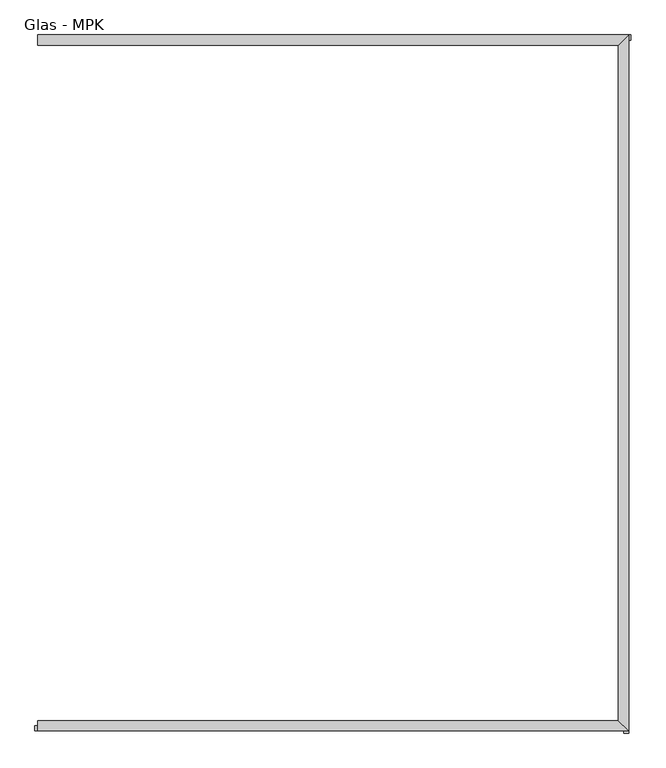
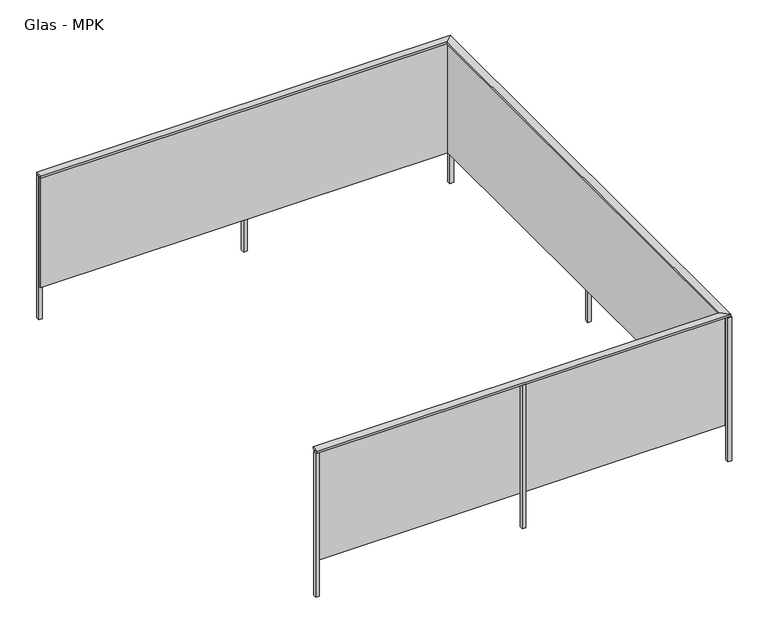
"""IFC4 building model written with IfcOpenShell, lengths in millimetres: railing geometry, Glas - MPK."""

from ifc_helpers import new_model, si_unit, frame, origin, place, context, project, spatial, polyline, outline, extrude, faceted_brep, source, transform, mapped, element, save


def glas_mpk_c28c6285(model_context):
    return source(origin(), model_context, "Body", "SolidModel", [
        faceted_brep([(29194.1667192, -1196.642277, 3843.2628643), (29194.1667192, -1246.642277, 3843.2628643), (29194.1667192, -1246.642277, 3856.7371357), (29194.1667192, -1196.642277, 3856.7371357), (32034.1667192, -1196.642277, 3843.2628643), (31984.1667192, -1246.642277, 3843.2628643), (31984.1667192, -1246.642277, 3856.7371357), (32034.1667192, -1196.642277, 3856.7371357), (32034.1667192, -4537.3716232, 3843.2628643), (31984.1667192, -4487.3716232, 3843.2628643), (31984.1667192, -4487.3716232, 3856.7371357), (32034.1667192, -4537.3716232, 3856.7371357), (29194.1667192, -4537.3716232, 3843.2628643), (29194.1667192, -4537.3716232, 3856.7371357), (29194.1667192, -4487.3716232, 3856.7371357), (29194.1667192, -4487.3716232, 3843.2628643)], [[[0, 1, 2, 3]], [[1, 0, 4, 5]], [[2, 1, 5, 6]], [[3, 2, 6, 7]], [[0, 3, 7, 4]], [[5, 4, 8, 9]], [[6, 5, 9, 10]], [[7, 6, 10, 11]], [[4, 7, 11, 8]], [[12, 13, 14, 15]], [[9, 8, 12, 15]], [[10, 9, 15, 14]], [[11, 10, 14, 13]], [[8, 11, 13, 12]]]),
        faceted_brep([(29194.1667192, -1236.642277, 3842.8769824), (29194.1667192, -1222.4501531, 3842.8769824), (29194.1667192, -1222.4501531, 3042.8769824), (29194.1667192, -1236.642277, 3042.8769824), (31994.1667192, -1236.642277, 3842.8769824), (32008.3588432, -1222.4501531, 3842.8769824), (32008.3588432, -1222.4501531, 3042.8769824), (31994.1667192, -1236.642277, 3042.8769824), (31994.1667192, -4497.3716232, 3842.8769824), (32008.3588432, -4511.5637472, 3842.8769824), (32008.3588432, -4511.5637472, 3042.8769824), (31994.1667192, -4497.3716232, 3042.8769824), (29194.1667192, -4497.3716232, 3842.8769824), (29194.1667192, -4497.3716232, 3042.8769824), (29194.1667192, -4511.5637472, 3042.8769824), (29194.1667192, -4511.5637472, 3842.8769824)], [[[0, 1, 2, 3]], [[1, 0, 4, 5]], [[2, 1, 5, 6]], [[3, 2, 6, 7]], [[0, 3, 7, 4]], [[5, 4, 8, 9]], [[6, 5, 9, 10]], [[7, 6, 10, 11]], [[4, 7, 11, 8]], [[12, 13, 14, 15]], [[9, 8, 12, 15]], [[10, 9, 15, 14]], [[11, 10, 14, 13]], [[8, 11, 13, 12]]]),
        extrude(outline(polyline([(30625.4167192, -4512.3716232), (30625.4167192, -4537.3716232), (30600.4167192, -4537.3716232), (30600.4167192, -4512.3716232), (30625.4167192, -4512.3716232)])), frame((0.0, 0.0, 2800.0), z_axis=(0.0, 0.0, 1.0), x_axis=(1.0, 0.0, 0.0)), (0.0, 0.0, 1.0), 1043.2628643),
        extrude(outline(polyline([(32009.1667192, -2854.5069501), (32034.1667192, -2854.5069501), (32034.1667192, -2879.5069501), (32009.1667192, -2879.5069501), (32009.1667192, -2854.5069501)])), frame((0.0, 0.0, 2800.0), z_axis=(0.0, 0.0, 1.0), x_axis=(1.0, 0.0, 0.0)), (0.0, 0.0, 1.0), 1043.2628643),
        extrude(outline(polyline([(30600.4167192, -1221.642277), (30600.4167192, -1196.642277), (30625.4167192, -1196.642277), (30625.4167192, -1221.642277), (30600.4167192, -1221.642277)])), frame((0.0, 0.0, 2800.0), z_axis=(0.0, 0.0, 1.0), x_axis=(1.0, 0.0, 0.0)), (0.0, 0.0, 1.0), 1043.2628643),
        extrude(outline(polyline([(32009.1667192, -4522.3716232), (32034.1667192, -4522.3716232), (32034.1667192, -4547.3716232), (32009.1667192, -4547.3716232), (32009.1667192, -4522.3716232)])), frame((0.0, 0.0, 2800.0), z_axis=(0.0, 0.0, 1.0), x_axis=(1.0, 0.0, 0.0)), (0.0, 0.0, 1.0), 1043.2628643),
        extrude(outline(polyline([(32019.1667192, -1221.642277), (32019.1667192, -1196.642277), (32044.1667192, -1196.642277), (32044.1667192, -1221.642277), (32019.1667192, -1221.642277)])), frame((0.0, 0.0, 2800.0), z_axis=(0.0, 0.0, 1.0), x_axis=(1.0, 0.0, 0.0)), (0.0, 0.0, 1.0), 1043.2628643),
        extrude(outline(polyline([(29206.6667192, -4512.3716232), (29206.6667192, -4537.3716232), (29181.6667192, -4537.3716232), (29181.6667192, -4512.3716232), (29206.6667192, -4512.3716232)])), frame((0.0, 0.0, 2800.0), z_axis=(0.0, 0.0, 1.0), x_axis=(1.0, 0.0, 0.0)), (0.0, 0.0, 1.0), 1043.2628643),
        extrude(outline(polyline([(29194.1667192, -1221.642277), (29194.1667192, -1196.642277), (29219.1667192, -1196.642277), (29219.1667192, -1221.642277), (29194.1667192, -1221.642277)])), frame((0.0, 0.0, 2800.0), z_axis=(0.0, 0.0, 1.0), x_axis=(1.0, 0.0, 0.0)), (0.0, 0.0, 1.0), 1043.2628643),
    ])


if __name__ == "__main__":
    model = new_model("IFC4")
    model_context = context("Model", 3, world=origin())
    ifc_project = project(units=[si_unit("LENGTHUNIT", "METRE", prefix="MILLI")], contexts=[model_context])
    site = spatial("IfcSite", under=ifc_project)
    building = spatial("IfcBuilding", under=site)
    placement = place(None, origin())
    glas_mpk_shape = glas_mpk_c28c6285(model_context)
    element("IfcRailing", 1, ObjectType="Glas - MPK", at=placement, inside=building, context=model_context, shape_type="MappedRepresentation", body=[
        mapped(glas_mpk_shape, transform((0.0, 0.0, 0.0), x_axis=(1.0, 0.0, 0.0), y_axis=(0.0, 1.0, 0.0), z_axis=(0.0, 0.0, 1.0))),
    ])
    save(model, "model.ifc")

# Revit data of these elements
# Element 1 (IfcRailing, "Glas - MPK")
#   Materials on its faces: "Metal - Aluminum", "Window - Glass"
# Materials
#   "Metal - Aluminum": class "Unassigned", colour RGB 247 247 247, transparency 0, Comments = "Rendering appearance not upgraded "
#   "Window - Glass": class "Glas", colour RGB 128 128 255, transparency 0.75
